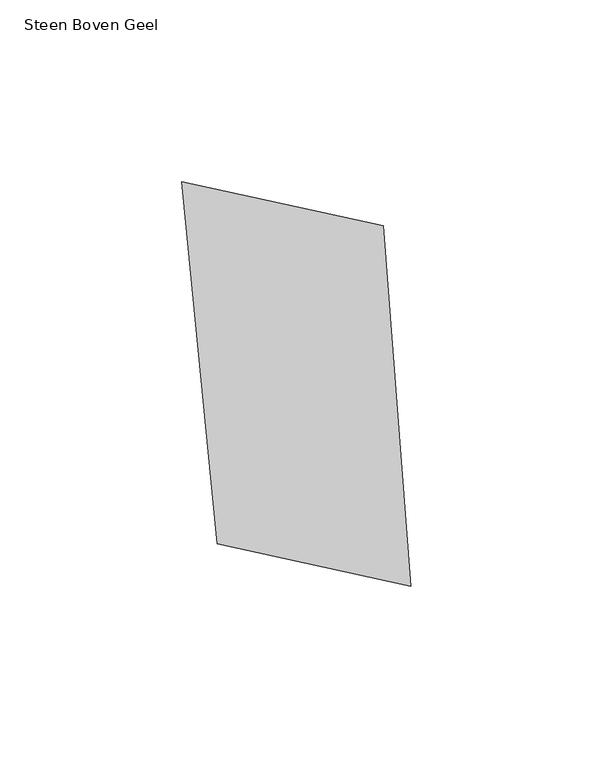
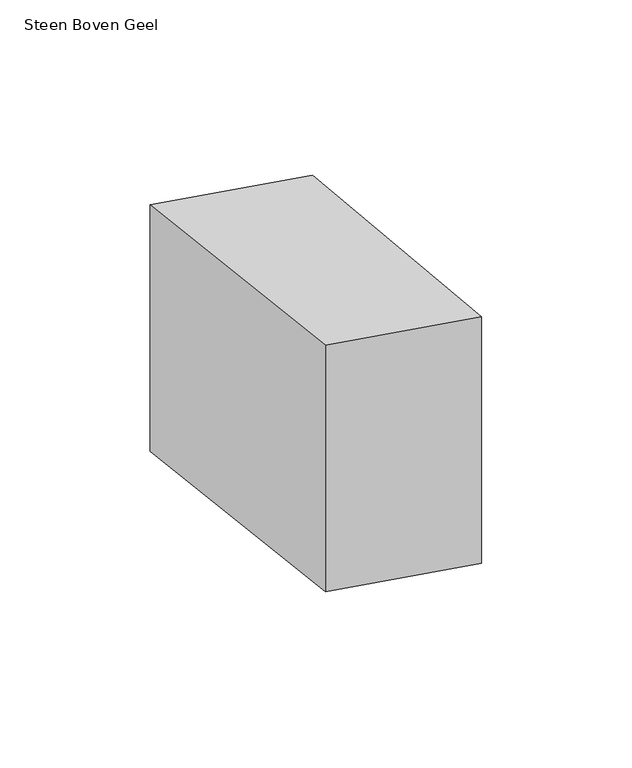
"""IFC4 building model written with IfcOpenShell, lengths in millimetres: proxy geometry, 00_GMA_steen_versie_4 : Steen Boven Geel."""

from ifc_helpers import new_model, si_unit, origin, origin_with_axes, place, context, project, spatial, polyline, outline, extrude, source, transform, mapped, element, save


def steen_boven_geel_110d0ab1(model_context):
    return source(origin(), model_context, "Body", "SweptSolid", [
        extrude(outline(polyline([(96.664914, 121.7093816), (104.287023, 22.5967349), (50.9926491, 34.191998), (41.2992654, 133.7823292), (96.664914, 121.7093816)])), origin_with_axes(), (0.0, 0.0, 1.0), 100.0),
    ])


if __name__ == "__main__":
    model = new_model("IFC4")
    model_context = context("Model", 3, world=origin())
    ifc_project = project(units=[si_unit("LENGTHUNIT", "METRE", prefix="MILLI")], contexts=[model_context])
    site = spatial("IfcSite", under=ifc_project)
    building = spatial("IfcBuilding", under=site)
    placement = place(None, origin())
    steen_boven_geel_shape = steen_boven_geel_110d0ab1(model_context)
    element("IfcBuildingElementProxy", 1, Name="00_GMA_steen_versie_4 : Steen Boven Geel", ObjectType="00_GMA_steen_versie_4 : Steen Boven Geel", at=placement, inside=building, context=model_context, shape_type="MappedRepresentation", body=[
        mapped(steen_boven_geel_shape, transform((0.0, 0.0, 0.0), x_axis=(1.0, 0.0, 0.0), y_axis=(0.0, 1.0, 0.0), z_axis=(0.0, 0.0, 1.0))),
    ])
    save(model, "model.ifc")

# Revit data of these elements
# Type "00_GMA_steen_versie_4 : Steen Boven Geel"
#   StootVoegHalfBoven [instance default] = 5 mm
#   StootVoegHalf [instance default] = 5 mm
#   StootVoegBreedteOnder = 10 mm
#   StootVoegBreedteBoven = 10 mm
#   Steendikte = 100 mm
#   LintVoegOnderHalf = 5 mm
#   LintVoegOnder = 10 mm
#   LintVoegBovenHalf = 0 mm
#   LintVoegBoven = 0 mm
#   materiaal = 21_steen_geel
#   MateriaalVoeg = none
#   Default Elevation = 0
# Element 1 (IfcBuildingElementProxy, "00_GMA_steen_versie_4 : Steen Boven Geel")
#   Materials on its faces: "21_steen_geel"
# Materials
#   "21_steen_geel": class "Unassigned", colour RGB 202 202 0, transparency 0, Cost = 0
